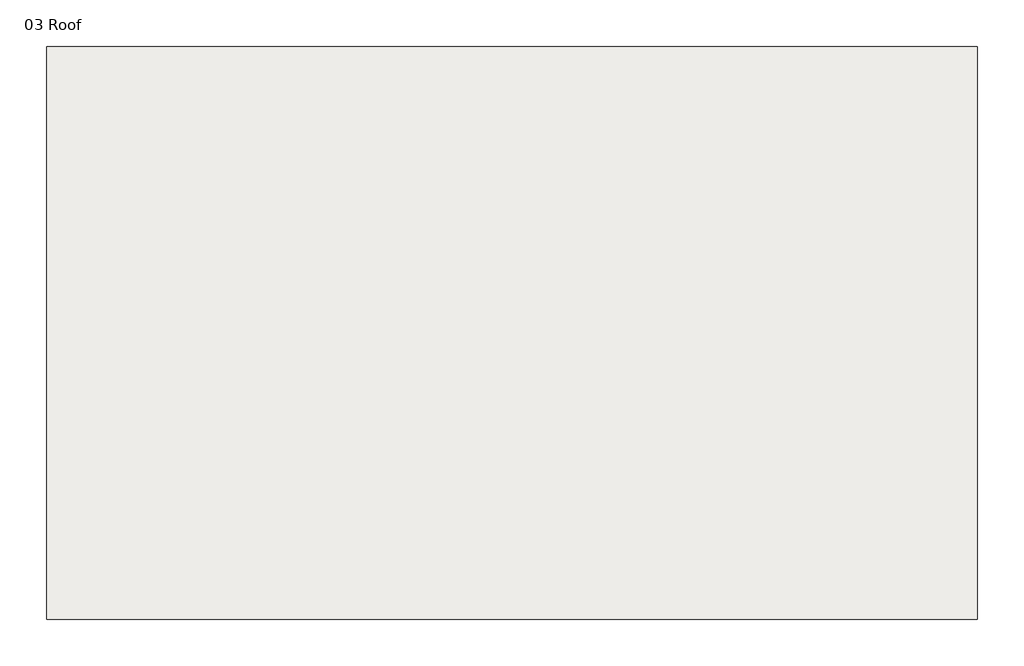
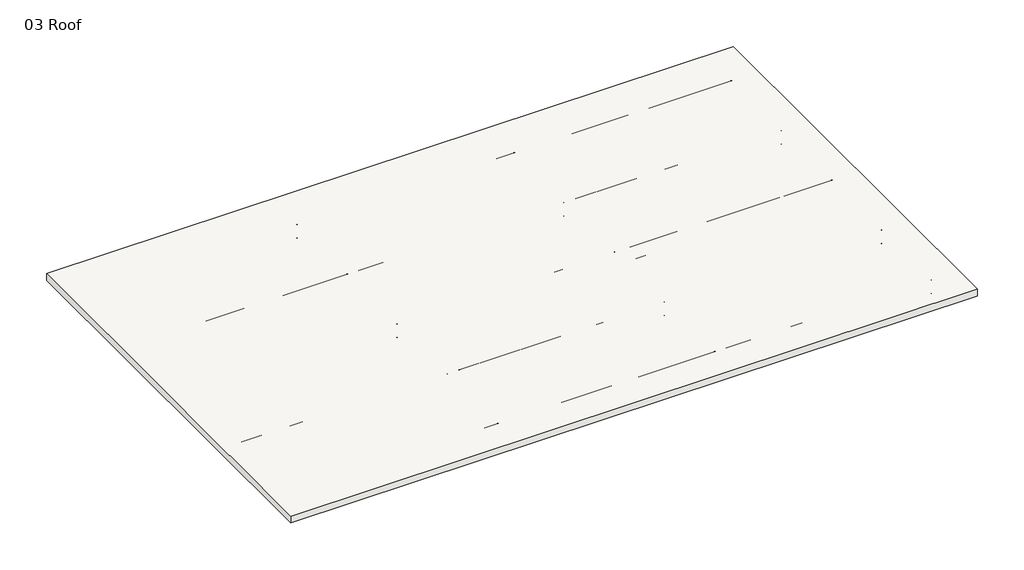
# One storey, part 1 of 4: 100 beams, 1 roof.
"""IFC4 building model written with IfcOpenShell, lengths in millimetres."""

import ifcopenshell
import ifcopenshell.guid

model = None  # the IFC model being written
_history = None  # IfcOwnerHistory: only IFC2X3 demands one
_inside = {}  # id of a spatial element -> (the spatial element, [elements in it])
_under = {}  # id of a project, library or spatial element -> (it, [spatial elements below it])
_declared = {}  # id of a project -> (the project, [libraries it declares])
_typed = {}  # id of a type object -> (the type object, [elements of that type])
_made_of = {}  # id of a material, layer set ... -> (it, [elements and type objects made of it])


def new_model(schema):
    """Start an empty IFC model of exactly this schema.

    Asked for "IFC4X3", IfcOpenShell would pick the latest addendum, in which some entities
    have other attributes; the version numbers below select the first issue.
    IFC2X3 requires an IfcOwnerHistory on every rooted entity: one is made here for all.
    """
    global model, _history
    if schema == "IFC4X3":
        model = ifcopenshell.file(schema_version=(4, 3, 0, 0))
    else:
        model = ifcopenshell.file(schema=schema)
    _inside.clear()
    _under.clear()
    _declared.clear()
    _typed.clear()
    _made_of.clear()
    _history = None
    if model.schema == "IFC2X3":
        org = make("IfcOrganization", Name="unknown")
        user = make(
            "IfcPersonAndOrganization",
            ThePerson=make("IfcPerson", FamilyName="unknown"),
            TheOrganization=org,
        )
        app = make(
            "IfcApplication",
            ApplicationDeveloper=org,
            Version="unknown",
            ApplicationFullName="unknown",
            ApplicationIdentifier="unknown",
        )
        _history = make(
            "IfcOwnerHistory",
            OwningUser=user,
            OwningApplication=app,
            ChangeAction="ADDED",
            CreationDate=0,
        )
    return model


def make(cls, **values):
    """One entity of the class cls with the attributes given. An attribute that is None is left unset."""
    return model.create_entity(
        cls, **{name: value for name, value in values.items() if value is not None}
    )


def rooted(cls, **values):
    """An entity with a GlobalId (a new one), such as an element, a storey or a relation."""
    return make(cls, GlobalId=ifcopenshell.guid.new(), OwnerHistory=_history, **values)


def si_unit(unit_type, name, prefix=None):
    """IfcSIUnit, for example si_unit("LENGTHUNIT", "METRE", prefix="MILLI")."""
    return make("IfcSIUnit", UnitType=unit_type, Prefix=prefix, Name=name)


def assignment(units):
    """IfcUnitAssignment: the units of a project."""
    return None if units is None else make("IfcUnitAssignment", Units=units)


def point(xyz):
    """IfcCartesianPoint."""
    return None if xyz is None else make("IfcCartesianPoint", Coordinates=xyz)


def direction(xyz):
    """IfcDirection."""
    return None if xyz is None else make("IfcDirection", DirectionRatios=xyz)


def frame(location, z_axis=None, x_axis=None):
    """IfcAxis2Placement3D, a coordinate frame: its origin and axes. An axis left out is left unset."""
    return make(
        "IfcAxis2Placement3D",
        Location=point(location),
        Axis=direction(z_axis),
        RefDirection=direction(x_axis),
    )


def frame_2d(location, x_axis=None):
    """IfcAxis2Placement2D, a coordinate frame in the plane: its origin and x axis."""
    return make(
        "IfcAxis2Placement2D", Location=point(location), RefDirection=direction(x_axis)
    )


def origin():
    """The frame at (0, 0, 0) with its axes left unset."""
    return frame((0.0, 0.0, 0.0))


def place(relative_to, where):
    """IfcLocalPlacement: puts the frame where relative to a parent placement (None: the world)."""
    return make(
        "IfcLocalPlacement", PlacementRelTo=relative_to, RelativePlacement=where
    )


def context(
    kind, dimensions, precision=None, world=None, true_north=None, identifier=None
):
    """IfcGeometricRepresentationContext, for example the 3D "Model" context."""
    return make(
        "IfcGeometricRepresentationContext",
        ContextIdentifier=identifier,
        ContextType=kind,
        CoordinateSpaceDimension=dimensions,
        Precision=precision,
        WorldCoordinateSystem=world,
        TrueNorth=true_north,
    )


def project(units=None, contexts=None):
    """IfcProject with its units and contexts."""
    return rooted(
        "IfcProject",
        Name="project",
        RepresentationContexts=contexts,
        UnitsInContext=assignment(units),
    )


def spatial(cls, under=None, at=None, **own):
    """A site, building, storey or space (cls), placed at a placement, below another one or the project."""
    s = rooted(cls, ObjectPlacement=at, **own)
    if under is not None:
        _under.setdefault(under.id(), (under, []))[1].append(s)
    return s


def polyline(points):
    """IfcPolyline through the points."""
    return make("IfcPolyline", Points=[point(p) for p in points])


def circle_curve(where, radius):
    """IfcCircle in the frame where."""
    return make("IfcCircle", Position=where, Radius=radius)


def trimmed(basis, trim1, trim2, sense, master):
    """IfcTrimmedCurve: the piece of a basis curve between two trims."""
    return make(
        "IfcTrimmedCurve",
        BasisCurve=basis,
        Trim1=trim1,
        Trim2=trim2,
        SenseAgreement=sense,
        MasterRepresentation=master,
    )


def segment(curve, same_sense, transition):
    """IfcCompositeCurveSegment."""
    return make(
        "IfcCompositeCurveSegment",
        Transition=transition,
        SameSense=same_sense,
        ParentCurve=curve,
    )


def composite_curve(segments, self_intersect=None):
    """IfcCompositeCurve: segments joined end to end."""
    return make("IfcCompositeCurve", Segments=segments, SelfIntersect=self_intersect)


def outline(outer, holes=None, kind="AREA"):
    """IfcArbitraryClosedProfileDef: a profile drawn as a closed curve; with holes, ...WithVoids."""
    if holes is None:
        return make("IfcArbitraryClosedProfileDef", ProfileType=kind, OuterCurve=outer)
    return make(
        "IfcArbitraryProfileDefWithVoids",
        ProfileType=kind,
        OuterCurve=outer,
        InnerCurves=holes,
    )


def extrude(swept, where, along, depth):
    """IfcExtrudedAreaSolid: the profile swept, set in the frame where, extruded along a direction by depth."""
    return make(
        "IfcExtrudedAreaSolid",
        SweptArea=swept,
        Position=where,
        ExtrudedDirection=direction(along),
        Depth=depth,
    )


def shape(context_of_items, identifier, shape_type, items):
    """IfcShapeRepresentation: the items that make up one representation, for example the "Body"."""
    return make(
        "IfcShapeRepresentation",
        ContextOfItems=context_of_items,
        RepresentationIdentifier=identifier,
        RepresentationType=shape_type,
        Items=items,
    )


def source(mapping_origin, context_of_items, identifier, shape_type, items):
    """IfcRepresentationMap: a shape defined once, which mapped items show again and again."""
    return make(
        "IfcRepresentationMap",
        MappingOrigin=mapping_origin,
        MappedRepresentation=shape(context_of_items, identifier, shape_type, items),
    )


def transform(
    local_origin,
    x_axis=None,
    y_axis=None,
    z_axis=None,
    scale=None,
    scale2=None,
    scale3=None,
    uniform=True,
):
    """IfcCartesianTransformationOperator3D, or its non-uniform kind. x_axis, y_axis, z_axis: its Axis1, 2, 3."""
    if uniform:
        return make(
            "IfcCartesianTransformationOperator3D",
            Axis1=direction(x_axis),
            Axis2=direction(y_axis),
            LocalOrigin=point(local_origin),
            Scale=scale,
            Axis3=direction(z_axis),
        )
    return make(
        "IfcCartesianTransformationOperator3DnonUniform",
        Axis1=direction(x_axis),
        Axis2=direction(y_axis),
        LocalOrigin=point(local_origin),
        Scale=scale,
        Axis3=direction(z_axis),
        Scale2=scale2,
        Scale3=scale3,
    )


def mapped(mapping_source, mapping_target):
    """IfcMappedItem: shows the shape of a source again, moved by a transform."""
    return make(
        "IfcMappedItem", MappingSource=mapping_source, MappingTarget=mapping_target
    )


def made_of(thing, what):
    """Note that an element or type object is made of a material, layer set ...; save() writes the relation."""
    if what is not None:
        _made_of.setdefault(what.id(), (what, []))[1].append(thing)
    return thing


def element(
    cls,
    number,
    at=None,
    inside=None,
    cuts=None,
    type_object=None,
    material=None,
    context=None,
    identifier="Body",
    shape_type=None,
    held_by="IfcProductDefinitionShape",
    body=None,
    shapes=None,
    **own,
):
    """One element of the class cls, such as IfcWall. Its Tag is "e" and its number.

    at: its placement. inside: the storey or other place that contains it. cuts: it is an
    opening in that element (IfcRelVoidsElement). A single representation is given by context,
    identifier, shape_type and body (its items); several are given by shapes. held_by: the class
    of the entity that holds the representations. save() writes the other relations.
    """
    e = rooted(cls, Tag="e%d" % number, ObjectPlacement=at, **own)
    if body is not None:
        shapes = [shape(context, identifier, shape_type, body)]
    if shapes is not None:
        e.Representation = make(held_by, Representations=shapes)
    if inside is not None:
        _inside.setdefault(inside.id(), (inside, []))[1].append(e)
    if cuts is not None:
        rooted(
            "IfcRelVoidsElement", RelatingBuildingElement=cuts, RelatedOpeningElement=e
        )
    if type_object is not None:
        _typed.setdefault(type_object.id(), (type_object, []))[1].append(e)
    return made_of(e, material)


def aggregate(whole, parts):
    """IfcRelAggregates: a whole, such as a stair, and the parts it consists of."""
    return rooted("IfcRelAggregates", RelatingObject=whole, RelatedObjects=parts)


def save(model, path):
    """Write the relations noted so far, then the file.

    IfcRelAggregates (storeys below a building ...), IfcRelContainedInSpatialStructure (elements
    in a storey), IfcRelDefinesByType, IfcRelAssociatesMaterial and IfcRelDeclares: one each for
    every whole, place, type object, material and project.
    """
    for whole, parts in _under.values():
        aggregate(whole, parts)
    for where, things in _inside.values():
        rooted(
            "IfcRelContainedInSpatialStructure",
            RelatedElements=things,
            RelatingStructure=where,
        )
    for kind, things in _typed.values():
        rooted("IfcRelDefinesByType", RelatedObjects=things, RelatingType=kind)
    for what, things in _made_of.values():
        rooted("IfcRelAssociatesMaterial", RelatedObjects=things, RelatingMaterial=what)
    for by, libraries in _declared.values():
        rooted("IfcRelDeclares", RelatingContext=by, RelatedDefinitions=libraries)
    model.write(path)


def ub_universal_beam_305x165x40ub_24de31be(model_context):
    return source(origin(), model_context, "Body", "SweptSolid", [
        extrude(outline(composite_curve([segment(polyline([(82.5, -141.5), (82.5, -151.7), (-82.5, -151.7), (-82.5, -141.5), (-11.9, -141.5)]), True, "CONTINUOUS"), segment(trimmed(circle_curve(frame_2d((-11.9, -132.6)), 8.9), [point((-11.9, -141.5))], [point((-3.0, -132.6))], True, "CARTESIAN"), True, "CONTINUOUS"), segment(polyline([(-3.0, -132.6), (-3.0, 132.6)]), True, "CONTINUOUS"), segment(trimmed(circle_curve(frame_2d((-11.9, 132.6)), 8.9), [point((-3.0, 132.6))], [point((-11.9, 141.5))], True, "CARTESIAN"), True, "CONTINUOUS"), segment(polyline([(-11.9, 141.5), (-82.5, 141.5), (-82.5, 151.7), (82.5, 151.7), (82.5, 141.5), (11.9, 141.5)]), True, "CONTINUOUS"), segment(trimmed(circle_curve(frame_2d((11.9, 132.6)), 8.9), [point((11.9, 141.5))], [point((3.0, 132.6))], True, "CARTESIAN"), True, "CONTINUOUS"), segment(polyline([(3.0, 132.6), (3.0, -132.6)]), True, "CONTINUOUS"), segment(trimmed(circle_curve(frame_2d((11.9, -132.6)), 8.9), [point((3.0, -132.6))], [point((11.9, -141.5))], True, "CARTESIAN"), True, "CONTINUOUS"), segment(polyline([(11.9, -141.5), (82.5, -141.5)]), True, "CONTINUOUS")], self_intersect=False)), frame((-335.6, 0.0, 0.0), z_axis=(1.0, 0.0, 0.0), x_axis=(0.0, 1.0, 0.0)), (0.0, 0.0, 1.0), 671.2),
    ])


def ub_universal_beam_305x165x40ub_f67fc52f(model_context):
    return source(origin(), model_context, "Body", "SweptSolid", [
        extrude(outline(composite_curve([segment(polyline([(82.5, -141.5), (82.5, -151.7), (-82.5, -151.7), (-82.5, -141.5), (-11.9, -141.5)]), True, "CONTINUOUS"), segment(trimmed(circle_curve(frame_2d((-11.9, -132.6)), 8.9), [point((-11.9, -141.5))], [point((-3.0, -132.6))], True, "CARTESIAN"), True, "CONTINUOUS"), segment(polyline([(-3.0, -132.6), (-3.0, 132.6)]), True, "CONTINUOUS"), segment(trimmed(circle_curve(frame_2d((-11.9, 132.6)), 8.9), [point((-3.0, 132.6))], [point((-11.9, 141.5))], True, "CARTESIAN"), True, "CONTINUOUS"), segment(polyline([(-11.9, 141.5), (-82.5, 141.5), (-82.5, 151.7), (82.5, 151.7), (82.5, 141.5), (11.9, 141.5)]), True, "CONTINUOUS"), segment(trimmed(circle_curve(frame_2d((11.9, 132.6)), 8.9), [point((11.9, 141.5))], [point((3.0, 132.6))], True, "CARTESIAN"), True, "CONTINUOUS"), segment(polyline([(3.0, 132.6), (3.0, -132.6)]), True, "CONTINUOUS"), segment(trimmed(circle_curve(frame_2d((11.9, -132.6)), 8.9), [point((3.0, -132.6))], [point((11.9, -141.5))], True, "CARTESIAN"), True, "CONTINUOUS"), segment(polyline([(11.9, -141.5), (82.5, -141.5)]), True, "CONTINUOUS")], self_intersect=False)), frame((-7125.0, 0.0, 0.0), z_axis=(1.0, 0.0, 0.0), x_axis=(0.0, 1.0, 0.0)), (0.0, 0.0, 1.0), 14250.0),
    ])


def ub_universal_beam_305x165x40ub_26fb8d3a(model_context):
    return source(origin(), model_context, "Body", "SweptSolid", [
        extrude(outline(composite_curve([segment(polyline([(82.5, -141.5), (82.5, -151.7), (-82.5, -151.7), (-82.5, -141.5), (-11.9, -141.5)]), True, "CONTINUOUS"), segment(trimmed(circle_curve(frame_2d((-11.9, -132.6)), 8.9), [point((-11.9, -141.5))], [point((-3.0, -132.6))], True, "CARTESIAN"), True, "CONTINUOUS"), segment(polyline([(-3.0, -132.6), (-3.0, 132.6)]), True, "CONTINUOUS"), segment(trimmed(circle_curve(frame_2d((-11.9, 132.6)), 8.9), [point((-3.0, 132.6))], [point((-11.9, 141.5))], True, "CARTESIAN"), True, "CONTINUOUS"), segment(polyline([(-11.9, 141.5), (-82.5, 141.5), (-82.5, 151.7), (82.5, 151.7), (82.5, 141.5), (11.9, 141.5)]), True, "CONTINUOUS"), segment(trimmed(circle_curve(frame_2d((11.9, 132.6)), 8.9), [point((11.9, 141.5))], [point((3.0, 132.6))], True, "CARTESIAN"), True, "CONTINUOUS"), segment(polyline([(3.0, 132.6), (3.0, -132.6)]), True, "CONTINUOUS"), segment(trimmed(circle_curve(frame_2d((11.9, -132.6)), 8.9), [point((3.0, -132.6))], [point((11.9, -141.5))], True, "CARTESIAN"), True, "CONTINUOUS"), segment(polyline([(11.9, -141.5), (82.5, -141.5)]), True, "CONTINUOUS")], self_intersect=False)), frame((-347.8807825, 0.0, 0.0), z_axis=(1.0, 0.0, 0.0), x_axis=(0.0, 1.0, 0.0)), (0.0, 0.0, 1.0), 695.761565),
    ])


model = new_model("IFC4")

# Units and contexts
model_context = context("Model", 3, world=origin())
ifc_project = project(units=[si_unit("LENGTHUNIT", "METRE", prefix="MILLI")], contexts=[model_context])

# Site, building, storey
site = spatial("IfcSite", under=ifc_project)
building = spatial("IfcBuilding", under=site)
storey = spatial("IfcBuildingStorey", under=building, Name="03 Roof", Elevation=8000.0)

# Beams
placement = place(None, origin())
ub_universal_beam_305x165x40ub_shape = ub_universal_beam_305x165x40ub_24de31be(model_context)
element("IfcBeam", 1, ObjectType="UB-Universal Beam : 305x165x40UB", at=placement, inside=storey, context=model_context, shape_type="MappedRepresentation", body=[
    mapped(ub_universal_beam_305x165x40ub_shape, transform((8848.4493174, -11728.1525129, 7500.0), x_axis=(0.0, 0.0, 1.0), y_axis=(0.0, -1.0, 0.0), z_axis=(1.0, 0.0, 0.0))),
])
element("IfcBeam", 2, ObjectType="UB-Universal Beam : 305x165x40UB", at=placement, inside=storey, context=model_context, shape_type="MappedRepresentation", body=[
    mapped(ub_universal_beam_305x165x40ub_shape, transform((7660.9493174, -11728.1525129, 7500.0), x_axis=(0.0, 0.0, 1.0), y_axis=(0.0, -1.0, 0.0), z_axis=(1.0, 0.0, 0.0))),
])
element("IfcBeam", 3, ObjectType="UB-Universal Beam : 305x165x40UB", at=placement, inside=storey, context=model_context, shape_type="MappedRepresentation", body=[
    mapped(ub_universal_beam_305x165x40ub_shape, transform((-6151.5506826, -5728.1525129, 7500.0), x_axis=(0.0, 0.0, 1.0), y_axis=(0.0, -1.0, 0.0), z_axis=(1.0, 0.0, 0.0))),
])
element("IfcBeam", 4, ObjectType="UB-Universal Beam : 305x165x40UB", at=placement, inside=storey, context=model_context, shape_type="MappedRepresentation", body=[
    mapped(ub_universal_beam_305x165x40ub_shape, transform((-4964.0506826, -5728.1525129, 7500.0), x_axis=(0.0, 0.0, 1.0), y_axis=(0.0, -1.0, 0.0), z_axis=(1.0, 0.0, 0.0))),
])
element("IfcBeam", 5, ObjectType="UB-Universal Beam : 305x165x40UB", at=placement, inside=storey, context=model_context, shape_type="MappedRepresentation", body=[
    mapped(ub_universal_beam_305x165x40ub_shape, transform((-3776.5506826, -5728.1525129, 7500.0), x_axis=(0.0, 0.0, 1.0), y_axis=(0.0, -1.0, 0.0), z_axis=(1.0, 0.0, 0.0))),
])
element("IfcBeam", 6, ObjectType="UB-Universal Beam : 305x165x40UB", at=placement, inside=storey, context=model_context, shape_type="MappedRepresentation", body=[
    mapped(ub_universal_beam_305x165x40ub_shape, transform((-2589.0506826, -5728.1525129, 7500.0), x_axis=(0.0, 0.0, 1.0), y_axis=(0.0, -1.0, 0.0), z_axis=(1.0, 0.0, 0.0))),
])
element("IfcBeam", 7, ObjectType="UB-Universal Beam : 305x165x40UB", at=placement, inside=storey, context=model_context, shape_type="MappedRepresentation", body=[
    mapped(ub_universal_beam_305x165x40ub_shape, transform((-7339.0506826, -5728.1525129, 7500.0), x_axis=(0.0, 0.0, 1.0), y_axis=(0.0, -1.0, 0.0), z_axis=(1.0, 0.0, 0.0))),
])
element("IfcBeam", 8, ObjectType="UB-Universal Beam : 305x165x40UB", at=placement, inside=storey, context=model_context, shape_type="MappedRepresentation", body=[
    mapped(ub_universal_beam_305x165x40ub_shape, transform((-1401.5506826, -5728.1525129, 7500.0), x_axis=(0.0, 0.0, 1.0), y_axis=(0.0, -1.0, 0.0), z_axis=(1.0, 0.0, 0.0))),
])
element("IfcBeam", 9, ObjectType="UB-Universal Beam : 305x165x40UB", at=placement, inside=storey, context=model_context, shape_type="MappedRepresentation", body=[
    mapped(ub_universal_beam_305x165x40ub_shape, transform((-214.0506826, -5728.1525129, 7500.0), x_axis=(0.0, 0.0, 1.0), y_axis=(0.0, -1.0, 0.0), z_axis=(1.0, 0.0, 0.0))),
])
element("IfcBeam", 10, ObjectType="UB-Universal Beam : 305x165x40UB", at=placement, inside=storey, context=model_context, shape_type="MappedRepresentation", body=[
    mapped(ub_universal_beam_305x165x40ub_shape, transform((5723.4493174, -11728.1525129, 7500.0), x_axis=(0.0, 0.0, 1.0), y_axis=(0.0, -1.0, 0.0), z_axis=(1.0, 0.0, 0.0))),
])
element("IfcBeam", 11, ObjectType="UB-Universal Beam : 305x165x40UB", at=placement, inside=storey, context=model_context, shape_type="MappedRepresentation", body=[
    mapped(ub_universal_beam_305x165x40ub_shape, transform((-6151.5506826, -11728.1525129, 7500.0), x_axis=(0.0, 0.0, 1.0), y_axis=(0.0, -1.0, 0.0), z_axis=(1.0, 0.0, 0.0))),
])
element("IfcBeam", 12, ObjectType="UB-Universal Beam : 305x165x40UB", at=placement, inside=storey, context=model_context, shape_type="MappedRepresentation", body=[
    mapped(ub_universal_beam_305x165x40ub_shape, transform((4535.9493174, -11728.1525129, 7500.0), x_axis=(0.0, 0.0, 1.0), y_axis=(0.0, -1.0, 0.0), z_axis=(1.0, 0.0, 0.0))),
])
element("IfcBeam", 13, ObjectType="UB-Universal Beam : 305x165x40UB", at=placement, inside=storey, context=model_context, shape_type="MappedRepresentation", body=[
    mapped(ub_universal_beam_305x165x40ub_shape, transform((-4964.0506826, -11728.1525129, 7500.0), x_axis=(0.0, 0.0, 1.0), y_axis=(0.0, -1.0, 0.0), z_axis=(1.0, 0.0, 0.0))),
])
element("IfcBeam", 14, ObjectType="UB-Universal Beam : 305x165x40UB", at=placement, inside=storey, context=model_context, shape_type="MappedRepresentation", body=[
    mapped(ub_universal_beam_305x165x40ub_shape, transform((3348.4493174, -11728.1525129, 7500.0), x_axis=(0.0, 0.0, 1.0), y_axis=(0.0, -1.0, 0.0), z_axis=(1.0, 0.0, 0.0))),
])
element("IfcBeam", 15, ObjectType="UB-Universal Beam : 305x165x40UB", at=placement, inside=storey, context=model_context, shape_type="MappedRepresentation", body=[
    mapped(ub_universal_beam_305x165x40ub_shape, transform((2160.9493174, -11728.1525129, 7500.0), x_axis=(0.0, 0.0, 1.0), y_axis=(0.0, -1.0, 0.0), z_axis=(1.0, 0.0, 0.0))),
])
element("IfcBeam", 16, ObjectType="UB-Universal Beam : 305x165x40UB", at=placement, inside=storey, context=model_context, shape_type="MappedRepresentation", body=[
    mapped(ub_universal_beam_305x165x40ub_shape, transform((6910.9493174, -11728.1525129, 7500.0), x_axis=(0.0, 0.0, 1.0), y_axis=(0.0, -1.0, 0.0), z_axis=(1.0, 0.0, 0.0))),
])
element("IfcBeam", 17, ObjectType="UB-Universal Beam : 305x165x40UB", at=placement, inside=storey, context=model_context, shape_type="MappedRepresentation", body=[
    mapped(ub_universal_beam_305x165x40ub_shape, transform((973.4493174, -11728.1525129, 7500.0), x_axis=(0.0, 0.0, 1.0), y_axis=(0.0, -1.0, 0.0), z_axis=(1.0, 0.0, 0.0))),
])
element("IfcBeam", 18, ObjectType="UB-Universal Beam : 305x165x40UB", at=placement, inside=storey, context=model_context, shape_type="MappedRepresentation", body=[
    mapped(ub_universal_beam_305x165x40ub_shape, transform((-3776.5506826, -11728.1525129, 7500.0), x_axis=(0.0, 0.0, 1.0), y_axis=(0.0, -1.0, 0.0), z_axis=(1.0, 0.0, 0.0))),
])
element("IfcBeam", 19, ObjectType="UB-Universal Beam : 305x165x40UB", at=placement, inside=storey, context=model_context, shape_type="MappedRepresentation", body=[
    mapped(ub_universal_beam_305x165x40ub_shape, transform((-2589.0506826, -11728.1525129, 7500.0), x_axis=(0.0, 0.0, 1.0), y_axis=(0.0, -1.0, 0.0), z_axis=(1.0, 0.0, 0.0))),
])
element("IfcBeam", 20, ObjectType="UB-Universal Beam : 305x165x40UB", at=placement, inside=storey, context=model_context, shape_type="MappedRepresentation", body=[
    mapped(ub_universal_beam_305x165x40ub_shape, transform((-7339.0506826, -11728.1525129, 7500.0), x_axis=(0.0, 0.0, 1.0), y_axis=(0.0, -1.0, 0.0), z_axis=(1.0, 0.0, 0.0))),
])
element("IfcBeam", 21, ObjectType="UB-Universal Beam : 305x165x40UB", at=placement, inside=storey, context=model_context, shape_type="MappedRepresentation", body=[
    mapped(ub_universal_beam_305x165x40ub_shape, transform((-1401.5506826, -11728.1525129, 7500.0), x_axis=(0.0, 0.0, 1.0), y_axis=(0.0, -1.0, 0.0), z_axis=(1.0, 0.0, 0.0))),
])
element("IfcBeam", 22, ObjectType="UB-Universal Beam : 305x165x40UB", at=placement, inside=storey, context=model_context, shape_type="MappedRepresentation", body=[
    mapped(ub_universal_beam_305x165x40ub_shape, transform((-214.0506826, -11728.1525129, 7500.0), x_axis=(0.0, 0.0, 1.0), y_axis=(0.0, -1.0, 0.0), z_axis=(1.0, 0.0, 0.0))),
])
element("IfcBeam", 23, ObjectType="UB-Universal Beam : 305x165x40UB", at=placement, inside=storey, context=model_context, shape_type="MappedRepresentation", body=[
    mapped(ub_universal_beam_305x165x40ub_shape, transform((-9276.5506826, -5728.1525129, 7500.0), x_axis=(0.0, 0.0, 1.0), y_axis=(0.0, -1.0, 0.0), z_axis=(1.0, 0.0, 0.0))),
])
element("IfcBeam", 24, ObjectType="UB-Universal Beam : 305x165x40UB", at=placement, inside=storey, context=model_context, shape_type="MappedRepresentation", body=[
    mapped(ub_universal_beam_305x165x40ub_shape, transform((-21151.5506826, -5728.1525129, 7500.0), x_axis=(0.0, 0.0, 1.0), y_axis=(0.0, -1.0, 0.0), z_axis=(1.0, 0.0, 0.0))),
])
element("IfcBeam", 25, ObjectType="UB-Universal Beam : 305x165x40UB", at=placement, inside=storey, context=model_context, shape_type="MappedRepresentation", body=[
    mapped(ub_universal_beam_305x165x40ub_shape, transform((-10464.0506826, -5728.1525129, 7500.0), x_axis=(0.0, 0.0, 1.0), y_axis=(0.0, -1.0, 0.0), z_axis=(1.0, 0.0, 0.0))),
])
element("IfcBeam", 26, ObjectType="UB-Universal Beam : 305x165x40UB", at=placement, inside=storey, context=model_context, shape_type="MappedRepresentation", body=[
    mapped(ub_universal_beam_305x165x40ub_shape, transform((-19964.0506826, -5728.1525129, 7500.0), x_axis=(0.0, 0.0, 1.0), y_axis=(0.0, -1.0, 0.0), z_axis=(1.0, 0.0, 0.0))),
])
element("IfcBeam", 27, ObjectType="UB-Universal Beam : 305x165x40UB", at=placement, inside=storey, context=model_context, shape_type="MappedRepresentation", body=[
    mapped(ub_universal_beam_305x165x40ub_shape, transform((-11651.5506826, -5728.1525129, 7500.0), x_axis=(0.0, 0.0, 1.0), y_axis=(0.0, -1.0, 0.0), z_axis=(1.0, 0.0, 0.0))),
])
element("IfcBeam", 28, ObjectType="UB-Universal Beam : 305x165x40UB", at=placement, inside=storey, context=model_context, shape_type="MappedRepresentation", body=[
    mapped(ub_universal_beam_305x165x40ub_shape, transform((-12839.0506826, -5728.1525129, 7500.0), x_axis=(0.0, 0.0, 1.0), y_axis=(0.0, -1.0, 0.0), z_axis=(1.0, 0.0, 0.0))),
])
element("IfcBeam", 29, ObjectType="UB-Universal Beam : 305x165x40UB", at=placement, inside=storey, context=model_context, shape_type="MappedRepresentation", body=[
    mapped(ub_universal_beam_305x165x40ub_shape, transform((-8089.0506826, -5728.1525129, 7500.0), x_axis=(0.0, 0.0, 1.0), y_axis=(0.0, -1.0, 0.0), z_axis=(1.0, 0.0, 0.0))),
])
element("IfcBeam", 30, ObjectType="UB-Universal Beam : 305x165x40UB", at=placement, inside=storey, context=model_context, shape_type="MappedRepresentation", body=[
    mapped(ub_universal_beam_305x165x40ub_shape, transform((-14026.5506826, -5728.1525129, 7500.0), x_axis=(0.0, 0.0, 1.0), y_axis=(0.0, -1.0, 0.0), z_axis=(1.0, 0.0, 0.0))),
])
element("IfcBeam", 31, ObjectType="UB-Universal Beam : 305x165x40UB", at=placement, inside=storey, context=model_context, shape_type="MappedRepresentation", body=[
    mapped(ub_universal_beam_305x165x40ub_shape, transform((-18776.5506826, -5728.1525129, 7500.0), x_axis=(0.0, 0.0, 1.0), y_axis=(0.0, -1.0, 0.0), z_axis=(1.0, 0.0, 0.0))),
])
element("IfcBeam", 32, ObjectType="UB-Universal Beam : 305x165x40UB", at=placement, inside=storey, context=model_context, shape_type="MappedRepresentation", body=[
    mapped(ub_universal_beam_305x165x40ub_shape, transform((-17589.0506826, -5728.1525129, 7500.0), x_axis=(0.0, 0.0, 1.0), y_axis=(0.0, -1.0, 0.0), z_axis=(1.0, 0.0, 0.0))),
])
element("IfcBeam", 33, ObjectType="UB-Universal Beam : 305x165x40UB", at=placement, inside=storey, context=model_context, shape_type="MappedRepresentation", body=[
    mapped(ub_universal_beam_305x165x40ub_shape, transform((-22339.0506826, -5728.1525129, 7500.0), x_axis=(0.0, 0.0, 1.0), y_axis=(0.0, -1.0, 0.0), z_axis=(1.0, 0.0, 0.0))),
])
element("IfcBeam", 34, ObjectType="UB-Universal Beam : 305x165x40UB", at=placement, inside=storey, context=model_context, shape_type="MappedRepresentation", body=[
    mapped(ub_universal_beam_305x165x40ub_shape, transform((-16401.5506826, -5728.1525129, 7500.0), x_axis=(0.0, 0.0, 1.0), y_axis=(0.0, -1.0, 0.0), z_axis=(1.0, 0.0, 0.0))),
])
element("IfcBeam", 35, ObjectType="UB-Universal Beam : 305x165x40UB", at=placement, inside=storey, context=model_context, shape_type="MappedRepresentation", body=[
    mapped(ub_universal_beam_305x165x40ub_shape, transform((-15214.0506826, -5728.1525129, 7500.0), x_axis=(0.0, 0.0, 1.0), y_axis=(0.0, -1.0, 0.0), z_axis=(1.0, 0.0, 0.0))),
])
element("IfcBeam", 36, ObjectType="UB-Universal Beam : 305x165x40UB", at=placement, inside=storey, context=model_context, shape_type="MappedRepresentation", body=[
    mapped(ub_universal_beam_305x165x40ub_shape, transform((-9276.5506826, -11728.1525129, 7500.0), x_axis=(0.0, 0.0, 1.0), y_axis=(0.0, -1.0, 0.0), z_axis=(1.0, 0.0, 0.0))),
])
element("IfcBeam", 37, ObjectType="UB-Universal Beam : 305x165x40UB", at=placement, inside=storey, context=model_context, shape_type="MappedRepresentation", body=[
    mapped(ub_universal_beam_305x165x40ub_shape, transform((-21151.5506826, -11728.1525129, 7500.0), x_axis=(0.0, 0.0, 1.0), y_axis=(0.0, -1.0, 0.0), z_axis=(1.0, 0.0, 0.0))),
])
element("IfcBeam", 38, ObjectType="UB-Universal Beam : 305x165x40UB", at=placement, inside=storey, context=model_context, shape_type="MappedRepresentation", body=[
    mapped(ub_universal_beam_305x165x40ub_shape, transform((-10464.0506826, -11728.1525129, 7500.0), x_axis=(0.0, 0.0, 1.0), y_axis=(0.0, -1.0, 0.0), z_axis=(1.0, 0.0, 0.0))),
])
element("IfcBeam", 39, ObjectType="UB-Universal Beam : 305x165x40UB", at=placement, inside=storey, context=model_context, shape_type="MappedRepresentation", body=[
    mapped(ub_universal_beam_305x165x40ub_shape, transform((-19964.0506826, -11728.1525129, 7500.0), x_axis=(0.0, 0.0, 1.0), y_axis=(0.0, -1.0, 0.0), z_axis=(1.0, 0.0, 0.0))),
])
element("IfcBeam", 40, ObjectType="UB-Universal Beam : 305x165x40UB", at=placement, inside=storey, context=model_context, shape_type="MappedRepresentation", body=[
    mapped(ub_universal_beam_305x165x40ub_shape, transform((-11651.5506826, -11728.1525129, 7500.0), x_axis=(0.0, 0.0, 1.0), y_axis=(0.0, -1.0, 0.0), z_axis=(1.0, 0.0, 0.0))),
])
element("IfcBeam", 41, ObjectType="UB-Universal Beam : 305x165x40UB", at=placement, inside=storey, context=model_context, shape_type="MappedRepresentation", body=[
    mapped(ub_universal_beam_305x165x40ub_shape, transform((-12839.0506826, -11728.1525129, 7500.0), x_axis=(0.0, 0.0, 1.0), y_axis=(0.0, -1.0, 0.0), z_axis=(1.0, 0.0, 0.0))),
])
element("IfcBeam", 42, ObjectType="UB-Universal Beam : 305x165x40UB", at=placement, inside=storey, context=model_context, shape_type="MappedRepresentation", body=[
    mapped(ub_universal_beam_305x165x40ub_shape, transform((-8089.0506826, -11728.1525129, 7500.0), x_axis=(0.0, 0.0, 1.0), y_axis=(0.0, -1.0, 0.0), z_axis=(1.0, 0.0, 0.0))),
])
element("IfcBeam", 43, ObjectType="UB-Universal Beam : 305x165x40UB", at=placement, inside=storey, context=model_context, shape_type="MappedRepresentation", body=[
    mapped(ub_universal_beam_305x165x40ub_shape, transform((-14026.5506826, -11728.1525129, 7500.0), x_axis=(0.0, 0.0, 1.0), y_axis=(0.0, -1.0, 0.0), z_axis=(1.0, 0.0, 0.0))),
])
element("IfcBeam", 44, ObjectType="UB-Universal Beam : 305x165x40UB", at=placement, inside=storey, context=model_context, shape_type="MappedRepresentation", body=[
    mapped(ub_universal_beam_305x165x40ub_shape, transform((-18776.5506826, -11728.1525129, 7500.0), x_axis=(0.0, 0.0, 1.0), y_axis=(0.0, -1.0, 0.0), z_axis=(1.0, 0.0, 0.0))),
])
element("IfcBeam", 45, ObjectType="UB-Universal Beam : 305x165x40UB", at=placement, inside=storey, context=model_context, shape_type="MappedRepresentation", body=[
    mapped(ub_universal_beam_305x165x40ub_shape, transform((-17589.0506826, -11728.1525129, 7500.0), x_axis=(0.0, 0.0, 1.0), y_axis=(0.0, -1.0, 0.0), z_axis=(1.0, 0.0, 0.0))),
])
element("IfcBeam", 46, ObjectType="UB-Universal Beam : 305x165x40UB", at=placement, inside=storey, context=model_context, shape_type="MappedRepresentation", body=[
    mapped(ub_universal_beam_305x165x40ub_shape, transform((-22339.0506826, -11728.1525129, 7500.0), x_axis=(0.0, 0.0, 1.0), y_axis=(0.0, -1.0, 0.0), z_axis=(1.0, 0.0, 0.0))),
])
element("IfcBeam", 47, ObjectType="UB-Universal Beam : 305x165x40UB", at=placement, inside=storey, context=model_context, shape_type="MappedRepresentation", body=[
    mapped(ub_universal_beam_305x165x40ub_shape, transform((-16401.5506826, -11728.1525129, 7500.0), x_axis=(0.0, 0.0, 1.0), y_axis=(0.0, -1.0, 0.0), z_axis=(1.0, 0.0, 0.0))),
])
element("IfcBeam", 48, ObjectType="UB-Universal Beam : 305x165x40UB", at=placement, inside=storey, context=model_context, shape_type="MappedRepresentation", body=[
    mapped(ub_universal_beam_305x165x40ub_shape, transform((-15214.0506826, -11728.1525129, 7500.0), x_axis=(0.0, 0.0, 1.0), y_axis=(0.0, -1.0, 0.0), z_axis=(1.0, 0.0, 0.0))),
])
ub_universal_beam_305x165x40ub_2_shape = ub_universal_beam_305x165x40ub_f67fc52f(model_context)
element("IfcBeam", 49, ObjectType="UB-Universal Beam : 305x165x40UB", at=placement, inside=storey, context=model_context, shape_type="MappedRepresentation", body=[
    mapped(ub_universal_beam_305x165x40ub_2_shape, transform((-214.0506826, -5728.1525129, 7000.0), x_axis=(1.0, 0.0, 0.0), y_axis=(0.0, 1.0, 0.0), z_axis=(0.0, 0.0, 1.0))),
])
element("IfcBeam", 50, ObjectType="UB-Universal Beam : 305x165x40UB", at=placement, inside=storey, context=model_context, shape_type="MappedRepresentation", body=[
    mapped(ub_universal_beam_305x165x40ub_2_shape, transform((-214.0506826, -5728.1525129, 8000.0), x_axis=(1.0, 0.0, 0.0), y_axis=(0.0, 1.0, 0.0), z_axis=(0.0, 0.0, 1.0))),
])
element("IfcBeam", 51, ObjectType="UB-Universal Beam : 305x165x40UB", at=placement, inside=storey, context=model_context, shape_type="MappedRepresentation", body=[
    mapped(ub_universal_beam_305x165x40ub_2_shape, transform((-214.0506826, -11728.1525129, 7000.0), x_axis=(1.0, 0.0, 0.0), y_axis=(0.0, 1.0, 0.0), z_axis=(0.0, 0.0, 1.0))),
])
element("IfcBeam", 52, ObjectType="UB-Universal Beam : 305x165x40UB", at=placement, inside=storey, context=model_context, shape_type="MappedRepresentation", body=[
    mapped(ub_universal_beam_305x165x40ub_2_shape, transform((-214.0506826, -11728.1525129, 8000.0), x_axis=(1.0, 0.0, 0.0), y_axis=(0.0, 1.0, 0.0), z_axis=(0.0, 0.0, 1.0))),
])
element("IfcBeam", 53, ObjectType="UB-Universal Beam : 305x165x40UB", at=placement, inside=storey, context=model_context, shape_type="MappedRepresentation", body=[
    mapped(ub_universal_beam_305x165x40ub_2_shape, transform((-15214.0506826, -5728.1525129, 7000.0), x_axis=(1.0, 0.0, 0.0), y_axis=(0.0, 1.0, 0.0), z_axis=(0.0, 0.0, 1.0))),
])
element("IfcBeam", 54, ObjectType="UB-Universal Beam : 305x165x40UB", at=placement, inside=storey, context=model_context, shape_type="MappedRepresentation", body=[
    mapped(ub_universal_beam_305x165x40ub_2_shape, transform((-15214.0506826, -5728.1525129, 8000.0), x_axis=(1.0, 0.0, 0.0), y_axis=(0.0, 1.0, 0.0), z_axis=(0.0, 0.0, 1.0))),
])
element("IfcBeam", 55, ObjectType="UB-Universal Beam : 305x165x40UB", at=placement, inside=storey, context=model_context, shape_type="MappedRepresentation", body=[
    mapped(ub_universal_beam_305x165x40ub_2_shape, transform((-15214.0506826, -11728.1525129, 7000.0), x_axis=(1.0, 0.0, 0.0), y_axis=(0.0, 1.0, 0.0), z_axis=(0.0, 0.0, 1.0))),
])
element("IfcBeam", 56, ObjectType="UB-Universal Beam : 305x165x40UB", at=placement, inside=storey, context=model_context, shape_type="MappedRepresentation", body=[
    mapped(ub_universal_beam_305x165x40ub_2_shape, transform((-15214.0506826, -11728.1525129, 8000.0), x_axis=(1.0, 0.0, 0.0), y_axis=(0.0, 1.0, 0.0), z_axis=(0.0, 0.0, 1.0))),
])
ub_universal_beam_305x165x40ub_3_shape = ub_universal_beam_305x165x40ub_26fb8d3a(model_context)
element("IfcBeam", 57, ObjectType="UB-Universal Beam : 305x165x40UB", at=placement, inside=storey, context=model_context, shape_type="MappedRepresentation", body=[
    mapped(ub_universal_beam_305x165x40ub_3_shape, transform((9442.1993174, -11728.1525129, 7500.0), x_axis=(0.7649111981170519, 0.0, -0.6441357457827785), y_axis=(0.0, -1.0, 0.0), z_axis=(-0.6441357457827785, 0.0, -0.7649111981170519))),
])
element("IfcBeam", 58, ObjectType="UB-Universal Beam : 305x165x40UB", at=placement, inside=storey, context=model_context, shape_type="MappedRepresentation", body=[
    mapped(ub_universal_beam_305x165x40ub_3_shape, transform((8254.6993174, -11728.1525129, 7500.0), x_axis=(0.7649111981170554, 0.0, -0.6441357457827743), y_axis=(0.0, -1.0, 0.0), z_axis=(-0.6441357457827743, 0.0, -0.7649111981170554))),
])
element("IfcBeam", 59, ObjectType="UB-Universal Beam : 305x165x40UB", at=placement, inside=storey, context=model_context, shape_type="MappedRepresentation", body=[
    mapped(ub_universal_beam_305x165x40ub_3_shape, transform((-5557.8006826, -5728.1525129, 7500.0), x_axis=(0.7649111981170519, 0.0, -0.6441357457827785), y_axis=(0.0, -1.0, 0.0), z_axis=(-0.6441357457827785, 0.0, -0.7649111981170519))),
])
element("IfcBeam", 60, ObjectType="UB-Universal Beam : 305x165x40UB", at=placement, inside=storey, context=model_context, shape_type="MappedRepresentation", body=[
    mapped(ub_universal_beam_305x165x40ub_3_shape, transform((-4370.3006826, -5728.1525129, 7500.0), x_axis=(0.7649111981170512, 0.0, -0.6441357457827793), y_axis=(0.0, -1.0, 0.0), z_axis=(-0.6441357457827793, 0.0, -0.7649111981170512))),
])
element("IfcBeam", 61, ObjectType="UB-Universal Beam : 305x165x40UB", at=placement, inside=storey, context=model_context, shape_type="MappedRepresentation", body=[
    mapped(ub_universal_beam_305x165x40ub_3_shape, transform((-3182.8006826, -5728.1525129, 7500.0), x_axis=(0.7649111981170506, 0.0, -0.64413574578278), y_axis=(0.0, -1.0, 0.0), z_axis=(-0.64413574578278, 0.0, -0.7649111981170506))),
])
element("IfcBeam", 62, ObjectType="UB-Universal Beam : 305x165x40UB", at=placement, inside=storey, context=model_context, shape_type="MappedRepresentation", body=[
    mapped(ub_universal_beam_305x165x40ub_3_shape, transform((-1995.3006826, -5728.1525129, 7500.0), x_axis=(0.7649111981170498, 0.0, -0.644135745782781), y_axis=(0.0, -1.0, 0.0), z_axis=(-0.644135745782781, 0.0, -0.7649111981170498))),
])
element("IfcBeam", 63, ObjectType="UB-Universal Beam : 305x165x40UB", at=placement, inside=storey, context=model_context, shape_type="MappedRepresentation", body=[
    mapped(ub_universal_beam_305x165x40ub_3_shape, transform((-6745.3006826, -5728.1525129, 7500.0), x_axis=(0.7649111981170552, 0.0, -0.6441357457827747), y_axis=(0.0, -1.0, 0.0), z_axis=(-0.6441357457827747, 0.0, -0.7649111981170552))),
])
element("IfcBeam", 64, ObjectType="UB-Universal Beam : 305x165x40UB", at=placement, inside=storey, context=model_context, shape_type="MappedRepresentation", body=[
    mapped(ub_universal_beam_305x165x40ub_3_shape, transform((-807.8006826, -5728.1525129, 7500.0), x_axis=(0.7649111981170494, 0.0, -0.6441357457827815), y_axis=(0.0, -1.0, 0.0), z_axis=(-0.6441357457827815, 0.0, -0.7649111981170494))),
])
element("IfcBeam", 65, ObjectType="UB-Universal Beam : 305x165x40UB", at=placement, inside=storey, context=model_context, shape_type="MappedRepresentation", body=[
    mapped(ub_universal_beam_305x165x40ub_3_shape, transform((5129.6993174, -11728.1525129, 7500.0), x_axis=(0.7649111981170454, 0.0, 0.644135745782786), y_axis=(0.0, -1.0, 0.0), z_axis=(0.644135745782786, 0.0, -0.7649111981170454))),
])
element("IfcBeam", 66, ObjectType="UB-Universal Beam : 305x165x40UB", at=placement, inside=storey, context=model_context, shape_type="MappedRepresentation", body=[
    mapped(ub_universal_beam_305x165x40ub_3_shape, transform((-5557.8006826, -11728.1525129, 7500.0), x_axis=(0.7649111981170519, 0.0, -0.6441357457827785), y_axis=(0.0, -1.0, 0.0), z_axis=(-0.6441357457827785, 0.0, -0.7649111981170519))),
])
element("IfcBeam", 67, ObjectType="UB-Universal Beam : 305x165x40UB", at=placement, inside=storey, context=model_context, shape_type="MappedRepresentation", body=[
    mapped(ub_universal_beam_305x165x40ub_3_shape, transform((3942.1993174, -11728.1525129, 7500.0), x_axis=(0.7649111981170463, 0.0, 0.6441357457827852), y_axis=(0.0, -1.0, 0.0), z_axis=(0.6441357457827852, 0.0, -0.7649111981170463))),
])
element("IfcBeam", 68, ObjectType="UB-Universal Beam : 305x165x40UB", at=placement, inside=storey, context=model_context, shape_type="MappedRepresentation", body=[
    mapped(ub_universal_beam_305x165x40ub_3_shape, transform((-4370.3006826, -11728.1525129, 7500.0), x_axis=(0.7649111981170512, 0.0, -0.6441357457827793), y_axis=(0.0, -1.0, 0.0), z_axis=(-0.6441357457827793, 0.0, -0.7649111981170512))),
])
element("IfcBeam", 69, ObjectType="UB-Universal Beam : 305x165x40UB", at=placement, inside=storey, context=model_context, shape_type="MappedRepresentation", body=[
    mapped(ub_universal_beam_305x165x40ub_3_shape, transform((2754.6993174, -11728.1525129, 7500.0), x_axis=(0.7649111981170467, 0.0, 0.6441357457827848), y_axis=(0.0, -1.0, 0.0), z_axis=(0.6441357457827848, 0.0, -0.7649111981170467))),
])
element("IfcBeam", 70, ObjectType="UB-Universal Beam : 305x165x40UB", at=placement, inside=storey, context=model_context, shape_type="MappedRepresentation", body=[
    mapped(ub_universal_beam_305x165x40ub_3_shape, transform((1567.1993174, -11728.1525129, 7500.0), x_axis=(0.7649111981170473, 0.0, 0.6441357457827839), y_axis=(0.0, -1.0, 0.0), z_axis=(0.6441357457827839, 0.0, -0.7649111981170473))),
])
element("IfcBeam", 71, ObjectType="UB-Universal Beam : 305x165x40UB", at=placement, inside=storey, context=model_context, shape_type="MappedRepresentation", body=[
    mapped(ub_universal_beam_305x165x40ub_3_shape, transform((6317.1993174, -11728.1525129, 7500.0), x_axis=(0.7649111981170466, 0.0, 0.6441357457827848), y_axis=(0.0, -1.0, 0.0), z_axis=(0.6441357457827848, 0.0, -0.7649111981170466))),
])
element("IfcBeam", 72, ObjectType="UB-Universal Beam : 305x165x40UB", at=placement, inside=storey, context=model_context, shape_type="MappedRepresentation", body=[
    mapped(ub_universal_beam_305x165x40ub_3_shape, transform((379.6993174, -11728.1525129, 7500.0), x_axis=(0.764911198117048, 0.0, 0.6441357457827831), y_axis=(0.0, -1.0, 0.0), z_axis=(0.6441357457827831, 0.0, -0.764911198117048))),
])
element("IfcBeam", 73, ObjectType="UB-Universal Beam : 305x165x40UB", at=placement, inside=storey, context=model_context, shape_type="MappedRepresentation", body=[
    mapped(ub_universal_beam_305x165x40ub_3_shape, transform((-3182.8006826, -11728.1525129, 7500.0), x_axis=(0.7649111981170506, 0.0, -0.64413574578278), y_axis=(0.0, -1.0, 0.0), z_axis=(-0.64413574578278, 0.0, -0.7649111981170506))),
])
element("IfcBeam", 74, ObjectType="UB-Universal Beam : 305x165x40UB", at=placement, inside=storey, context=model_context, shape_type="MappedRepresentation", body=[
    mapped(ub_universal_beam_305x165x40ub_3_shape, transform((-1995.3006826, -11728.1525129, 7500.0), x_axis=(0.7649111981170498, 0.0, -0.644135745782781), y_axis=(0.0, -1.0, 0.0), z_axis=(-0.644135745782781, 0.0, -0.7649111981170498))),
])
element("IfcBeam", 75, ObjectType="UB-Universal Beam : 305x165x40UB", at=placement, inside=storey, context=model_context, shape_type="MappedRepresentation", body=[
    mapped(ub_universal_beam_305x165x40ub_3_shape, transform((-6745.3006826, -11728.1525129, 7500.0), x_axis=(0.7649111981170552, 0.0, -0.6441357457827747), y_axis=(0.0, -1.0, 0.0), z_axis=(-0.6441357457827747, 0.0, -0.7649111981170552))),
])
element("IfcBeam", 76, ObjectType="UB-Universal Beam : 305x165x40UB", at=placement, inside=storey, context=model_context, shape_type="MappedRepresentation", body=[
    mapped(ub_universal_beam_305x165x40ub_3_shape, transform((-807.8006826, -11728.1525129, 7500.0), x_axis=(0.7649111981170494, 0.0, -0.6441357457827815), y_axis=(0.0, -1.0, 0.0), z_axis=(-0.6441357457827815, 0.0, -0.7649111981170494))),
])
element("IfcBeam", 77, ObjectType="UB-Universal Beam : 305x165x40UB", at=placement, inside=storey, context=model_context, shape_type="MappedRepresentation", body=[
    mapped(ub_universal_beam_305x165x40ub_3_shape, transform((-9870.3006826, -5728.1525129, 7500.0), x_axis=(0.7649111981170454, 0.0, 0.644135745782786), y_axis=(0.0, -1.0, 0.0), z_axis=(0.644135745782786, 0.0, -0.7649111981170454))),
])
element("IfcBeam", 78, ObjectType="UB-Universal Beam : 305x165x40UB", at=placement, inside=storey, context=model_context, shape_type="MappedRepresentation", body=[
    mapped(ub_universal_beam_305x165x40ub_3_shape, transform((-20557.8006826, -5728.1525129, 7500.0), x_axis=(0.7649111981170519, 0.0, -0.6441357457827785), y_axis=(0.0, -1.0, 0.0), z_axis=(-0.6441357457827785, 0.0, -0.7649111981170519))),
])
element("IfcBeam", 79, ObjectType="UB-Universal Beam : 305x165x40UB", at=placement, inside=storey, context=model_context, shape_type="MappedRepresentation", body=[
    mapped(ub_universal_beam_305x165x40ub_3_shape, transform((-11057.8006826, -5728.1525129, 7500.0), x_axis=(0.7649111981170457, 0.0, 0.6441357457827859), y_axis=(0.0, -1.0, 0.0), z_axis=(0.6441357457827859, 0.0, -0.7649111981170457))),
])
element("IfcBeam", 80, ObjectType="UB-Universal Beam : 305x165x40UB", at=placement, inside=storey, context=model_context, shape_type="MappedRepresentation", body=[
    mapped(ub_universal_beam_305x165x40ub_3_shape, transform((-19370.3006826, -5728.1525129, 7500.0), x_axis=(0.7649111981170512, 0.0, -0.6441357457827793), y_axis=(0.0, -1.0, 0.0), z_axis=(-0.6441357457827793, 0.0, -0.7649111981170512))),
])
element("IfcBeam", 81, ObjectType="UB-Universal Beam : 305x165x40UB", at=placement, inside=storey, context=model_context, shape_type="MappedRepresentation", body=[
    mapped(ub_universal_beam_305x165x40ub_3_shape, transform((-12245.3006826, -5728.1525129, 7500.0), x_axis=(0.7649111981170463, 0.0, 0.6441357457827851), y_axis=(0.0, -1.0, 0.0), z_axis=(0.6441357457827851, 0.0, -0.7649111981170463))),
])
element("IfcBeam", 82, ObjectType="UB-Universal Beam : 305x165x40UB", at=placement, inside=storey, context=model_context, shape_type="MappedRepresentation", body=[
    mapped(ub_universal_beam_305x165x40ub_3_shape, transform((-13432.8006826, -5728.1525129, 7500.0), x_axis=(0.7649111981170482, 0.0, 0.6441357457827829), y_axis=(0.0, -1.0, 0.0), z_axis=(0.6441357457827829, 0.0, -0.7649111981170482))),
])
element("IfcBeam", 83, ObjectType="UB-Universal Beam : 305x165x40UB", at=placement, inside=storey, context=model_context, shape_type="MappedRepresentation", body=[
    mapped(ub_universal_beam_305x165x40ub_3_shape, transform((-8682.8006826, -5728.1525129, 7500.0), x_axis=(0.7649111981170466, 0.0, 0.6441357457827848), y_axis=(0.0, -1.0, 0.0), z_axis=(0.6441357457827848, 0.0, -0.7649111981170466))),
])
element("IfcBeam", 84, ObjectType="UB-Universal Beam : 305x165x40UB", at=placement, inside=storey, context=model_context, shape_type="MappedRepresentation", body=[
    mapped(ub_universal_beam_305x165x40ub_3_shape, transform((-14620.3006826, -5728.1525129, 7500.0), x_axis=(0.7649111981170483, 0.0, 0.6441357457827828), y_axis=(0.0, -1.0, 0.0), z_axis=(0.6441357457827828, 0.0, -0.7649111981170483))),
])
element("IfcBeam", 85, ObjectType="UB-Universal Beam : 305x165x40UB", at=placement, inside=storey, context=model_context, shape_type="MappedRepresentation", body=[
    mapped(ub_universal_beam_305x165x40ub_3_shape, transform((-18182.8006826, -5728.1525129, 7500.0), x_axis=(0.7649111981170511, 0.0, -0.6441357457827795), y_axis=(0.0, -1.0, 0.0), z_axis=(-0.6441357457827795, 0.0, -0.7649111981170511))),
])
element("IfcBeam", 86, ObjectType="UB-Universal Beam : 305x165x40UB", at=placement, inside=storey, context=model_context, shape_type="MappedRepresentation", body=[
    mapped(ub_universal_beam_305x165x40ub_3_shape, transform((-16995.3006826, -5728.1525129, 7500.0), x_axis=(0.7649111981170498, 0.0, -0.644135745782781), y_axis=(0.0, -1.0, 0.0), z_axis=(-0.644135745782781, 0.0, -0.7649111981170498))),
])
element("IfcBeam", 87, ObjectType="UB-Universal Beam : 305x165x40UB", at=placement, inside=storey, context=model_context, shape_type="MappedRepresentation", body=[
    mapped(ub_universal_beam_305x165x40ub_3_shape, transform((-21745.3006826, -5728.1525129, 7500.0), x_axis=(0.764911198117056, 0.0, -0.6441357457827737), y_axis=(0.0, -1.0, 0.0), z_axis=(-0.6441357457827737, 0.0, -0.764911198117056))),
])
element("IfcBeam", 88, ObjectType="UB-Universal Beam : 305x165x40UB", at=placement, inside=storey, context=model_context, shape_type="MappedRepresentation", body=[
    mapped(ub_universal_beam_305x165x40ub_3_shape, transform((-15807.8006826, -5728.1525129, 7500.0), x_axis=(0.7649111981170491, 0.0, -0.6441357457827819), y_axis=(0.0, -1.0, 0.0), z_axis=(-0.6441357457827819, 0.0, -0.7649111981170491))),
])
element("IfcBeam", 89, ObjectType="UB-Universal Beam : 305x165x40UB", at=placement, inside=storey, context=model_context, shape_type="MappedRepresentation", body=[
    mapped(ub_universal_beam_305x165x40ub_3_shape, transform((-9870.3006826, -11728.1525129, 7500.0), x_axis=(0.764911198117045, 0.0, 0.6441357457827868), y_axis=(0.0, -1.0, 0.0), z_axis=(0.6441357457827868, 0.0, -0.764911198117045))),
])
element("IfcBeam", 90, ObjectType="UB-Universal Beam : 305x165x40UB", at=placement, inside=storey, context=model_context, shape_type="MappedRepresentation", body=[
    mapped(ub_universal_beam_305x165x40ub_3_shape, transform((-20557.8006826, -11728.1525129, 7500.0), x_axis=(0.764911198117053, 0.0, -0.6441357457827771), y_axis=(0.0, -1.0, 0.0), z_axis=(-0.6441357457827771, 0.0, -0.764911198117053))),
])
element("IfcBeam", 91, ObjectType="UB-Universal Beam : 305x165x40UB", at=placement, inside=storey, context=model_context, shape_type="MappedRepresentation", body=[
    mapped(ub_universal_beam_305x165x40ub_3_shape, transform((-11057.8006826, -11728.1525129, 7500.0), x_axis=(0.7649111981170457, 0.0, 0.6441357457827859), y_axis=(0.0, -1.0, 0.0), z_axis=(0.6441357457827859, 0.0, -0.7649111981170457))),
])
element("IfcBeam", 92, ObjectType="UB-Universal Beam : 305x165x40UB", at=placement, inside=storey, context=model_context, shape_type="MappedRepresentation", body=[
    mapped(ub_universal_beam_305x165x40ub_3_shape, transform((-19370.3006826, -11728.1525129, 7500.0), x_axis=(0.7649111981170512, 0.0, -0.6441357457827793), y_axis=(0.0, -1.0, 0.0), z_axis=(-0.6441357457827793, 0.0, -0.7649111981170512))),
])
element("IfcBeam", 93, ObjectType="UB-Universal Beam : 305x165x40UB", at=placement, inside=storey, context=model_context, shape_type="MappedRepresentation", body=[
    mapped(ub_universal_beam_305x165x40ub_3_shape, transform((-12245.3006826, -11728.1525129, 7500.0), x_axis=(0.7649111981170463, 0.0, 0.6441357457827851), y_axis=(0.0, -1.0, 0.0), z_axis=(0.6441357457827851, 0.0, -0.7649111981170463))),
])
element("IfcBeam", 94, ObjectType="UB-Universal Beam : 305x165x40UB", at=placement, inside=storey, context=model_context, shape_type="MappedRepresentation", body=[
    mapped(ub_universal_beam_305x165x40ub_3_shape, transform((-13432.8006826, -11728.1525129, 7500.0), x_axis=(0.7649111981170477, 0.0, 0.6441357457827835), y_axis=(0.0, -1.0, 0.0), z_axis=(0.6441357457827835, 0.0, -0.7649111981170477))),
])
element("IfcBeam", 95, ObjectType="UB-Universal Beam : 305x165x40UB", at=placement, inside=storey, context=model_context, shape_type="MappedRepresentation", body=[
    mapped(ub_universal_beam_305x165x40ub_3_shape, transform((-8682.8006826, -11728.1525129, 7500.0), x_axis=(0.7649111981170466, 0.0, 0.6441357457827848), y_axis=(0.0, -1.0, 0.0), z_axis=(0.6441357457827848, 0.0, -0.7649111981170466))),
])
element("IfcBeam", 96, ObjectType="UB-Universal Beam : 305x165x40UB", at=placement, inside=storey, context=model_context, shape_type="MappedRepresentation", body=[
    mapped(ub_universal_beam_305x165x40ub_3_shape, transform((-14620.3006826, -11728.1525129, 7500.0), x_axis=(0.7649111981170483, 0.0, 0.6441357457827828), y_axis=(0.0, -1.0, 0.0), z_axis=(0.6441357457827828, 0.0, -0.7649111981170483))),
])
element("IfcBeam", 97, ObjectType="UB-Universal Beam : 305x165x40UB", at=placement, inside=storey, context=model_context, shape_type="MappedRepresentation", body=[
    mapped(ub_universal_beam_305x165x40ub_3_shape, transform((-18182.8006826, -11728.1525129, 7500.0), x_axis=(0.7649111981170504, 0.0, -0.6441357457827802), y_axis=(0.0, -1.0, 0.0), z_axis=(-0.6441357457827802, 0.0, -0.7649111981170504))),
])
element("IfcBeam", 98, ObjectType="UB-Universal Beam : 305x165x40UB", at=placement, inside=storey, context=model_context, shape_type="MappedRepresentation", body=[
    mapped(ub_universal_beam_305x165x40ub_3_shape, transform((-16995.3006826, -11728.1525129, 7500.0), x_axis=(0.7649111981170504, 0.0, -0.6441357457827803), y_axis=(0.0, -1.0, 0.0), z_axis=(-0.6441357457827803, 0.0, -0.7649111981170504))),
])
element("IfcBeam", 99, ObjectType="UB-Universal Beam : 305x165x40UB", at=placement, inside=storey, context=model_context, shape_type="MappedRepresentation", body=[
    mapped(ub_universal_beam_305x165x40ub_3_shape, transform((-21745.3006826, -11728.1525129, 7500.0), x_axis=(0.7649111981170549, 0.0, -0.644135745782775), y_axis=(0.0, -1.0, 0.0), z_axis=(-0.644135745782775, 0.0, -0.7649111981170549))),
])
element("IfcBeam", 100, ObjectType="UB-Universal Beam : 305x165x40UB", at=placement, inside=storey, context=model_context, shape_type="MappedRepresentation", body=[
    mapped(ub_universal_beam_305x165x40ub_3_shape, transform((-15807.8006826, -11728.1525129, 7500.0), x_axis=(0.7649111981170497, 0.0, -0.6441357457827811), y_axis=(0.0, -1.0, 0.0), z_axis=(-0.6441357457827811, 0.0, -0.7649111981170497))),
])

# Roof
element("IfcRoof", 101, ObjectType="Steel Bar Joist - Steel Deck - EPDM Membrane", at=placement, inside=storey, context=model_context, shape_type="SweptSolid", body=[
    extrude(outline(polyline([(-23939.0506826, 14871.8474871), (23510.9493174, 14871.8474871), (23510.9493174, -14353.1525129), (-23939.0506826, -14353.1525129), (-23939.0506826, 14871.8474871)])), frame((0.0, 0.0, 8000.0), z_axis=(0.0, 0.0, 1.0), x_axis=(1.0, 0.0, 0.0)), (0.0, 0.0, 1.0), 505.0),
])

save(model, "model.ifc")

# Revit data of these elements
# Project information
#   Project Issue Date = "October 2010"
#   Project Status = "Project Status"
#   Client Name = "Building CAD"
#   Project Address = "Enter address here"
#   Project Name = "Retail Units"
#   Project Number = "NA"
# Grids (mm)
#   "7.1": line (6910.949, -16246.876) -> (6910.949, 15788.475)
#   "4.2": line (-7339.051, -17601.714) -> (-7339.051, 15788.475)
#   "4.1": line (-8089.051, -16246.876) -> (-8089.051, 15788.475)
#   "7.2": line (7660.949, -17601.714) -> (7660.949, 15788.475)
#   "A.1": line (-26762.49, -12103.153) -> (24410.024, -12103.153)
#   "E.1": line (-27173.966, 12646.847) -> (26734.4, 12646.847)
#   "1.1": line (-22714.051, -16246.876) -> (-22714.051, 15788.475)
#   "10.1": line (22285.949, -16246.876) -> (22285.949, 15788.475)
#   "1": line (-22339.051, -14782.78) -> (-22339.051, 15788.475)
#   "2": line (-17714.051, -14782.78) -> (-17714.051, 15788.475)
#   "3": line (-12714.051, -14782.78) -> (-12714.051, 15788.475)
#   "4": line (-7714.051, -14782.78) -> (-7714.051, 15788.475)
#   "5": line (-2714.051, -14782.78) -> (-2714.051, 15788.475)
#   "6": line (2285.949, -14782.78) -> (2285.949, 15788.475)
#   "7": line (7285.949, -14782.78) -> (7285.949, 15788.475)
#   "8": line (12285.949, -14782.78) -> (12285.949, 15788.475)
#   "9": line (17285.949, -14782.78) -> (17285.949, 15788.475)
#   "10": line (21910.949, -14782.78) -> (21910.949, 15788.475)
#   "A": line (-25871.093, -11728.153) -> (26734.4, -11728.153)
#   "B": line (-25871.093, -5728.153) -> (26734.4, -5728.153)
#   "C": line (-25871.093, 271.847) -> (26734.4, 271.847)
#   "D": line (-25871.093, 6271.847) -> (26734.4, 6271.847)
#   "E": line (-25871.093, 12271.847) -> (26734.4, 12271.847)
# Type "UB-Universal Beam : 305x165x40UB"
#   Nominal h = "305"
#   W = 0
#   Start Extension Calculation [instance default] = 3000 mm
#   Start Extension [instance default] = -12.7 mm
#   End Extension Calculation [instance default] = 3000 mm
#   End Extension [instance default] = -12.7 mm
#   Ix = 8503
#   Length [instance default] = 1524 mm
#   M = 40.3
#   Zx = 560
#   b = 165 mm
#   h = 303.4 mm
#   r = 8.9 mm
#   s = 6 mm
#   t = 10.2 mm
#   A = 0.005 m²
#   Structural Material [instance default] = Metal - Steel - 345 MPa
#   Assembly Code = ""
# Type "Steel Bar Joist - Steel Deck - EPDM Membrane"
#   Layers, outside or top first: 5 mm "Roofing - EPDM Membrane" (function 4); 50 mm "Insulation / Thermal Barriers - Rigid insulation" (function 3); 50 mm "Metal - Decking" (function 1); 400 mm "Structure - Steel Bar Joist Layer" (function 1)
# Elements 1, 2, 3, 4, 5, 6, 7, 8, 9, 10, 11, 12, 13, 14, 15, 16, 17, 18, 19, 20, 21, 22, 23, 24, 25, 26, 27, 28, 29, 30, 31, 32, 33, 34, 35, 36, 37, 38, 39, 40, 41, 42, 43, 44, 45, 46, 47, 48, 49, 50, 51, 52, 53, 54, 55, 56, 57, 58, 59, 60, 61, 62, 63, 64, 65, 66, 67, 68, 69, 70, 71, 72, 73, 74, 75, 76, 77, 78, 79, 80, 81, 82, 83, 84, 85, 86, 87, 88, 89, 90, 91, 92, 93, 94, 95, 96, 97, 98, 99, 100 (IfcBeam, "UB-Universal Beam : 305x165x40UB")
#   Start Extension Calculation = 3000 mm
#   Start Extension = -12.7 mm
#   End Extension Calculation = 3000 mm
#   End Extension = -12.7 mm
#   Structural Material = Metal - Steel - 345 MPa
#   Phase Created = New Construction
#   Materials on its faces: "Metal - Steel - 345 MPa"
# Element 101 (IfcRoof, "Steel Bar Joist - Steel Deck - EPDM Membrane")
#   built-in parameter 1001705 = 27.9035 (stored number, unit not read)
#   built-in parameter 1001710 = 33615
#   Phase Created = New Construction
#   Materials on its faces: "Structure - Steel Bar Joist Layer", "Roofing - EPDM Membrane"
# Materials
#   "Metal - Steel - 345 MPa": class "Metal", colour RGB 241 46 46, transparency 0
#   "Roofing - EPDM Membrane": class "Plastic", colour RGB 127 127 127, transparency 0, Description = "Exterior finish, roofing"
#   "Insulation / Thermal Barriers - Rigid insulation": class "Miscellaneous", colour RGB 127 127 127, transparency 0
#   "Metal - Decking": class "Metal", colour RGB 247 247 247, transparency 0
#   "Structure - Steel Bar Joist Layer": class "Metal", colour RGB 127 127 127, transparency 0
